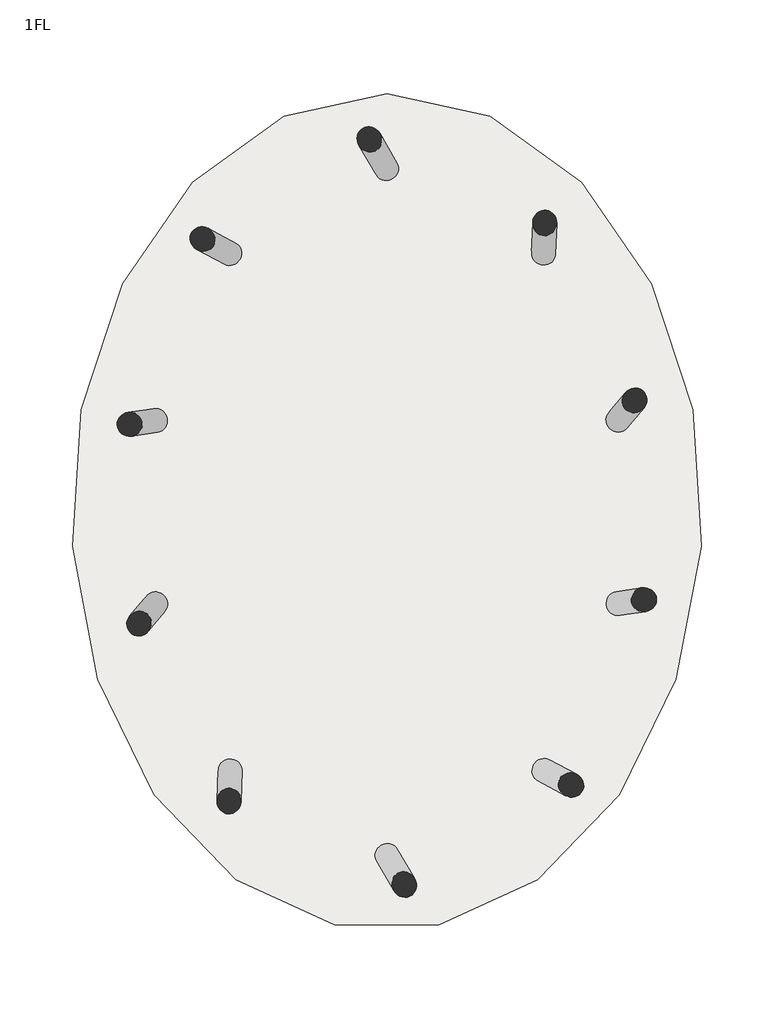
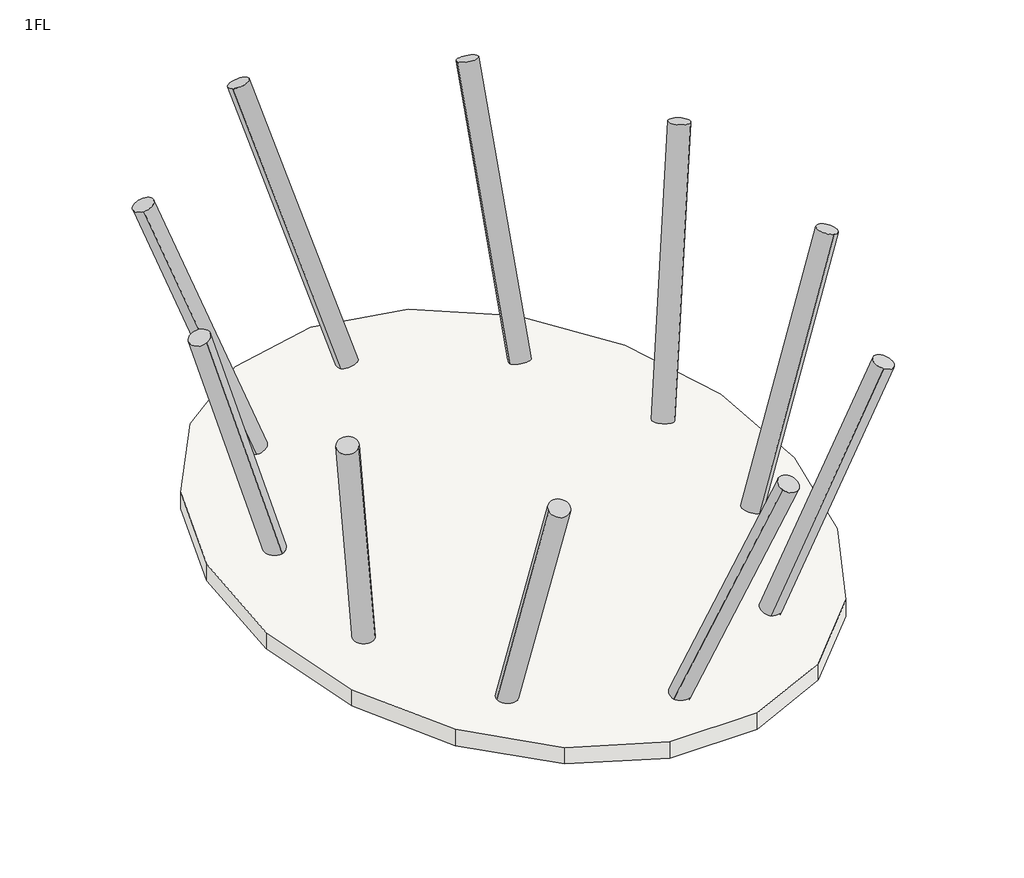
# One storey: 10 columns, 1 slab.
"""IFC4 building model written with IfcOpenShell, lengths in millimetres."""

import ifcopenshell
import ifcopenshell.guid

model = None  # the IFC model being written
_history = None  # IfcOwnerHistory: only IFC2X3 demands one
_inside = {}  # id of a spatial element -> (the spatial element, [elements in it])
_under = {}  # id of a project, library or spatial element -> (it, [spatial elements below it])
_declared = {}  # id of a project -> (the project, [libraries it declares])
_typed = {}  # id of a type object -> (the type object, [elements of that type])
_made_of = {}  # id of a material, layer set ... -> (it, [elements and type objects made of it])


def new_model(schema):
    """Start an empty IFC model of exactly this schema.

    Asked for "IFC4X3", IfcOpenShell would pick the latest addendum, in which some entities
    have other attributes; the version numbers below select the first issue.
    IFC2X3 requires an IfcOwnerHistory on every rooted entity: one is made here for all.
    """
    global model, _history
    if schema == "IFC4X3":
        model = ifcopenshell.file(schema_version=(4, 3, 0, 0))
    else:
        model = ifcopenshell.file(schema=schema)
    _inside.clear()
    _under.clear()
    _declared.clear()
    _typed.clear()
    _made_of.clear()
    _history = None
    if model.schema == "IFC2X3":
        org = make("IfcOrganization", Name="unknown")
        user = make(
            "IfcPersonAndOrganization",
            ThePerson=make("IfcPerson", FamilyName="unknown"),
            TheOrganization=org,
        )
        app = make(
            "IfcApplication",
            ApplicationDeveloper=org,
            Version="unknown",
            ApplicationFullName="unknown",
            ApplicationIdentifier="unknown",
        )
        _history = make(
            "IfcOwnerHistory",
            OwningUser=user,
            OwningApplication=app,
            ChangeAction="ADDED",
            CreationDate=0,
        )
    return model


def make(cls, **values):
    """One entity of the class cls with the attributes given. An attribute that is None is left unset."""
    return model.create_entity(
        cls, **{name: value for name, value in values.items() if value is not None}
    )


def rooted(cls, **values):
    """An entity with a GlobalId (a new one), such as an element, a storey or a relation."""
    return make(cls, GlobalId=ifcopenshell.guid.new(), OwnerHistory=_history, **values)


def si_unit(unit_type, name, prefix=None):
    """IfcSIUnit, for example si_unit("LENGTHUNIT", "METRE", prefix="MILLI")."""
    return make("IfcSIUnit", UnitType=unit_type, Prefix=prefix, Name=name)


def assignment(units):
    """IfcUnitAssignment: the units of a project."""
    return None if units is None else make("IfcUnitAssignment", Units=units)


def point(xyz):
    """IfcCartesianPoint."""
    return None if xyz is None else make("IfcCartesianPoint", Coordinates=xyz)


def direction(xyz):
    """IfcDirection."""
    return None if xyz is None else make("IfcDirection", DirectionRatios=xyz)


def frame(location, z_axis=None, x_axis=None):
    """IfcAxis2Placement3D, a coordinate frame: its origin and axes. An axis left out is left unset."""
    return make(
        "IfcAxis2Placement3D",
        Location=point(location),
        Axis=direction(z_axis),
        RefDirection=direction(x_axis),
    )


def frame_2d(location, x_axis=None):
    """IfcAxis2Placement2D, a coordinate frame in the plane: its origin and x axis."""
    return make(
        "IfcAxis2Placement2D", Location=point(location), RefDirection=direction(x_axis)
    )


def origin():
    """The frame at (0, 0, 0) with its axes left unset."""
    return frame((0.0, 0.0, 0.0))


def place(relative_to, where):
    """IfcLocalPlacement: puts the frame where relative to a parent placement (None: the world)."""
    return make(
        "IfcLocalPlacement", PlacementRelTo=relative_to, RelativePlacement=where
    )


def context(
    kind, dimensions, precision=None, world=None, true_north=None, identifier=None
):
    """IfcGeometricRepresentationContext, for example the 3D "Model" context."""
    return make(
        "IfcGeometricRepresentationContext",
        ContextIdentifier=identifier,
        ContextType=kind,
        CoordinateSpaceDimension=dimensions,
        Precision=precision,
        WorldCoordinateSystem=world,
        TrueNorth=true_north,
    )


def project(units=None, contexts=None):
    """IfcProject with its units and contexts."""
    return rooted(
        "IfcProject",
        Name="project",
        RepresentationContexts=contexts,
        UnitsInContext=assignment(units),
    )


def spatial(cls, under=None, at=None, **own):
    """A site, building, storey or space (cls), placed at a placement, below another one or the project."""
    s = rooted(cls, ObjectPlacement=at, **own)
    if under is not None:
        _under.setdefault(under.id(), (under, []))[1].append(s)
    return s


def polyline(points):
    """IfcPolyline through the points."""
    return make("IfcPolyline", Points=[point(p) for p in points])


def circle_curve(where, radius):
    """IfcCircle in the frame where."""
    return make("IfcCircle", Position=where, Radius=radius)


def trimmed(basis, trim1, trim2, sense, master):
    """IfcTrimmedCurve: the piece of a basis curve between two trims."""
    return make(
        "IfcTrimmedCurve",
        BasisCurve=basis,
        Trim1=trim1,
        Trim2=trim2,
        SenseAgreement=sense,
        MasterRepresentation=master,
    )


def segment(curve, same_sense, transition):
    """IfcCompositeCurveSegment."""
    return make(
        "IfcCompositeCurveSegment",
        Transition=transition,
        SameSense=same_sense,
        ParentCurve=curve,
    )


def composite_curve(segments, self_intersect=None):
    """IfcCompositeCurve: segments joined end to end."""
    return make("IfcCompositeCurve", Segments=segments, SelfIntersect=self_intersect)


def outline(outer, holes=None, kind="AREA"):
    """IfcArbitraryClosedProfileDef: a profile drawn as a closed curve; with holes, ...WithVoids."""
    if holes is None:
        return make("IfcArbitraryClosedProfileDef", ProfileType=kind, OuterCurve=outer)
    return make(
        "IfcArbitraryProfileDefWithVoids",
        ProfileType=kind,
        OuterCurve=outer,
        InnerCurves=holes,
    )


def extrude(swept, where, along, depth):
    """IfcExtrudedAreaSolid: the profile swept, set in the frame where, extruded along a direction by depth."""
    return make(
        "IfcExtrudedAreaSolid",
        SweptArea=swept,
        Position=where,
        ExtrudedDirection=direction(along),
        Depth=depth,
    )


def shape(context_of_items, identifier, shape_type, items):
    """IfcShapeRepresentation: the items that make up one representation, for example the "Body"."""
    return make(
        "IfcShapeRepresentation",
        ContextOfItems=context_of_items,
        RepresentationIdentifier=identifier,
        RepresentationType=shape_type,
        Items=items,
    )


def made_of(thing, what):
    """Note that an element or type object is made of a material, layer set ...; save() writes the relation."""
    if what is not None:
        _made_of.setdefault(what.id(), (what, []))[1].append(thing)
    return thing


def element(
    cls,
    number,
    at=None,
    inside=None,
    cuts=None,
    type_object=None,
    material=None,
    context=None,
    identifier="Body",
    shape_type=None,
    held_by="IfcProductDefinitionShape",
    body=None,
    shapes=None,
    **own,
):
    """One element of the class cls, such as IfcWall. Its Tag is "e" and its number.

    at: its placement. inside: the storey or other place that contains it. cuts: it is an
    opening in that element (IfcRelVoidsElement). A single representation is given by context,
    identifier, shape_type and body (its items); several are given by shapes. held_by: the class
    of the entity that holds the representations. save() writes the other relations.
    """
    e = rooted(cls, Tag="e%d" % number, ObjectPlacement=at, **own)
    if body is not None:
        shapes = [shape(context, identifier, shape_type, body)]
    if shapes is not None:
        e.Representation = make(held_by, Representations=shapes)
    if inside is not None:
        _inside.setdefault(inside.id(), (inside, []))[1].append(e)
    if cuts is not None:
        rooted(
            "IfcRelVoidsElement", RelatingBuildingElement=cuts, RelatedOpeningElement=e
        )
    if type_object is not None:
        _typed.setdefault(type_object.id(), (type_object, []))[1].append(e)
    return made_of(e, material)


def aggregate(whole, parts):
    """IfcRelAggregates: a whole, such as a stair, and the parts it consists of."""
    return rooted("IfcRelAggregates", RelatingObject=whole, RelatedObjects=parts)


def save(model, path):
    """Write the relations noted so far, then the file.

    IfcRelAggregates (storeys below a building ...), IfcRelContainedInSpatialStructure (elements
    in a storey), IfcRelDefinesByType, IfcRelAssociatesMaterial and IfcRelDeclares: one each for
    every whole, place, type object, material and project.
    """
    for whole, parts in _under.values():
        aggregate(whole, parts)
    for where, things in _inside.values():
        rooted(
            "IfcRelContainedInSpatialStructure",
            RelatedElements=things,
            RelatingStructure=where,
        )
    for kind, things in _typed.values():
        rooted("IfcRelDefinesByType", RelatedObjects=things, RelatingType=kind)
    for what, things in _made_of.values():
        rooted("IfcRelAssociatesMaterial", RelatedObjects=things, RelatingMaterial=what)
    for by, libraries in _declared.values():
        rooted("IfcRelDeclares", RelatingContext=by, RelatedDefinitions=libraries)
    model.write(path)


model = new_model("IFC4")

# Units and contexts
model_context = context("Model", 3, world=origin())
ifc_project = project(units=[si_unit("LENGTHUNIT", "METRE", prefix="MILLI")], contexts=[model_context])

# Site, building, storey
site = spatial("IfcSite", under=ifc_project)
building = spatial("IfcBuilding", under=site)
storey = spatial("IfcBuildingStorey", under=building, Name="1FL", Elevation=0.0)

# Columns
placement = place(None, origin())
element("IfcColumn", 1, ObjectType="コンクリート-円形-柱 : 750", at=placement, inside=storey, context=model_context, shape_type="SweptSolid", body=[
    extrude(outline(composite_curve([segment(trimmed(circle_curve(frame_2d((0.0, -175.0)), 175.0), [point((0.0, -350.0))], [point((0.0, 0.0))], False, "CARTESIAN"), True, "CONTINUOUS"), segment(trimmed(circle_curve(frame_2d((0.0, -175.0)), 175.0), [point((0.0, 0.0))], [point((0.0, -350.0))], False, "CARTESIAN"), True, "CONTINUOUS")], self_intersect=False)), frame((-150.9258136, 4911.4200994, 0.0), z_axis=(-0.19521767954583844, 0.33261932920084286, 0.9226345102123157), x_axis=(-0.46701070397496863, 0.7957106520636279, -0.3856754601543639)), (0.0, 0.0, 1.0), 4877.3376133),
])
element("IfcColumn", 2, ObjectType="コンクリート-円形-柱 : 750", at=placement, inside=storey, context=model_context, shape_type="SweptSolid", body=[
    extrude(outline(composite_curve([segment(trimmed(circle_curve(frame_2d((0.0, -175.0)), 175.0), [point((0.0, -350.0))], [point((0.0, 0.0))], False, "CARTESIAN"), True, "CONTINUOUS"), segment(trimmed(circle_curve(frame_2d((0.0, -175.0)), 175.0), [point((0.0, 0.0))], [point((0.0, -350.0))], False, "CARTESIAN"), True, "CONTINUOUS")], self_intersect=False)), frame((-2368.4341263, 3611.4937667, 0.0), z_axis=(-0.31275000049064827, 0.16672714276809913, 0.9350879622032815), x_axis=(-0.82515741745174, 0.43989172927194287, -0.3544157205070263)), (0.0, 0.0, 1.0), 4812.3814891),
])
element("IfcColumn", 3, ObjectType="コンクリート-円形-柱 : 750", at=placement, inside=storey, context=model_context, shape_type="SweptSolid", body=[
    extrude(outline(composite_curve([segment(trimmed(circle_curve(frame_2d((0.0, -175.0)), 175.0), [point((0.0, -350.0))], [point((0.0, 0.0))], False, "CARTESIAN"), True, "CONTINUOUS"), segment(trimmed(circle_curve(frame_2d((0.0, -175.0)), 175.0), [point((0.0, 0.0))], [point((0.0, -350.0))], False, "CARTESIAN"), True, "CONTINUOUS")], self_intersect=False)), frame((-3345.1996857, 1162.0255056, 0.0), z_axis=(-0.3023035165099614, -0.04397439962353301, 0.9521968473395936), x_axis=(-0.9422797649541056, -0.1370681605680071, -0.3054851287976858)), (0.0, 0.0, 1.0), 4725.9135677),
])
element("IfcColumn", 4, ObjectType="コンクリート-円形-柱 : 750", at=placement, inside=storey, context=model_context, shape_type="SweptSolid", body=[
    extrude(outline(composite_curve([segment(trimmed(circle_curve(frame_2d((0.0, -175.0)), 175.0), [point((0.0, -350.0))], [point((0.0, 0.0))], False, "CARTESIAN"), True, "CONTINUOUS"), segment(trimmed(circle_curve(frame_2d((0.0, -175.0)), 175.0), [point((0.0, 0.0))], [point((0.0, -350.0))], False, "CARTESIAN"), True, "CONTINUOUS")], self_intersect=False)), frame((-3236.0228376, -1447.3199745, 0.0), z_axis=(-0.19412294990655402, -0.23264885127893398, 0.9529904471284956), x_axis=(-0.6105515101907361, -0.7317223829581693, -0.3030003427090967)), (0.0, 0.0, 1.0), 4721.9780769),
])
element("IfcColumn", 5, ObjectType="コンクリート-円形-柱 : 750", at=placement, inside=storey, context=model_context, shape_type="SweptSolid", body=[
    extrude(outline(composite_curve([segment(trimmed(circle_curve(frame_2d((1e-07, -174.9999999)), 175.0), [point((0.0, -350.0))], [point((0.0, 0.0))], False, "CARTESIAN"), True, "CONTINUOUS"), segment(trimmed(circle_curve(frame_2d((1e-07, -174.9999999)), 175.0), [point((0.0, 0.0))], [point((0.0, -350.0))], False, "CARTESIAN"), True, "CONTINUOUS")], self_intersect=False)), frame((-2111.2371006, -3772.6097673, 0.0), z_axis=(-0.013415524296277117, -0.3507099157361099, 0.9363880492147616), x_axis=(-0.03579298830242224, -0.935703714164163, -0.3509664104836434)), (0.0, 0.0, 1.0), 4805.6999531),
])
element("IfcColumn", 6, ObjectType="コンクリート-円形-柱 : 750", at=placement, inside=storey, context=model_context, shape_type="SweptSolid", body=[
    extrude(outline(composite_curve([segment(trimmed(circle_curve(frame_2d((0.0, -175.0)), 175.0), [point((0.0, -349.9999999))], [point((0.0, 0.0))], False, "CARTESIAN"), True, "CONTINUOUS"), segment(trimmed(circle_curve(frame_2d((0.0, -175.0)), 175.0), [point((0.0, 0.0))], [point((0.0, -349.9999999))], False, "CARTESIAN"), True, "CONTINUOUS")], self_intersect=False)), frame((150.9258121, -4911.4201056, 0.0), z_axis=(0.19521768641578116, -0.332619328176475, 0.9226345091280188), x_axis=(0.46701071671984423, -0.7957106433262771, -0.3856754627482799)), (0.0, 0.0, 1.0), 4877.3376133),
])
element("IfcColumn", 7, ObjectType="コンクリート-円形-柱 : 750", at=placement, inside=storey, context=model_context, shape_type="SweptSolid", body=[
    extrude(outline(composite_curve([segment(trimmed(circle_curve(frame_2d((0.0, -175.0000001)), 175.0), [point((0.0, -350.0000001))], [point((0.0, 0.0))], False, "CARTESIAN"), True, "CONTINUOUS"), segment(trimmed(circle_curve(frame_2d((0.0, -175.0000001)), 175.0), [point((0.0, 0.0))], [point((0.0, -350.0000001))], False, "CARTESIAN"), True, "CONTINUOUS")], self_intersect=False)), frame((2368.4341596, -3611.4937481, 0.0), z_axis=(0.31274999648711344, -0.16672714070730643, 0.9350879639097471), x_axis=(0.8251574188770966, -0.439891730225705, -0.35441571600469896)), (0.0, 0.0, 1.0), 4812.3814891),
])
element("IfcColumn", 8, ObjectType="コンクリート-円形-柱 : 750", at=placement, inside=storey, context=model_context, shape_type="SweptSolid", body=[
    extrude(outline(composite_curve([segment(trimmed(circle_curve(frame_2d((-1e-07, -175.0000001)), 175.0), [point((0.0, -350.0))], [point((0.0, 0.0))], False, "CARTESIAN"), True, "CONTINUOUS"), segment(trimmed(circle_curve(frame_2d((-1e-07, -175.0000001)), 175.0), [point((0.0, 0.0))], [point((0.0, -350.0))], False, "CARTESIAN"), True, "CONTINUOUS")], self_intersect=False)), frame((3345.1996858, -1162.0254697, 0.0), z_axis=(0.30230351342511225, 0.04397439856797863, 0.9521968483677193), x_axis=(0.9422797662409613, 0.13706815886374568, -0.3054851255930188)), (0.0, 0.0, 1.0), 4725.9135677),
])
element("IfcColumn", 9, ObjectType="コンクリート-円形-柱 : 750", at=placement, inside=storey, context=model_context, shape_type="SweptSolid", body=[
    extrude(outline(composite_curve([segment(trimmed(circle_curve(frame_2d((0.0, -175.0)), 175.0), [point((0.0, -350.0))], [point((0.0, 0.0))], False, "CARTESIAN"), True, "CONTINUOUS"), segment(trimmed(circle_curve(frame_2d((0.0, -175.0)), 175.0), [point((0.0, 0.0))], [point((0.0, -350.0))], False, "CARTESIAN"), True, "CONTINUOUS")], self_intersect=False)), frame((3236.0228326, 1447.3200092, 0.0), z_axis=(0.19412294921583048, 0.23264884982996348, 0.9529904476229252), x_axis=(0.6105515114685474, 0.7317223825359012, -0.30300034115402713)), (0.0, 0.0, 1.0), 4721.9780769),
])
element("IfcColumn", 10, ObjectType="コンクリート-円形-柱 : 750", at=placement, inside=storey, context=model_context, shape_type="SweptSolid", body=[
    extrude(outline(composite_curve([segment(trimmed(circle_curve(frame_2d((-1e-07, -174.9999999)), 175.0), [point((-1e-07, -349.9999999))], [point((0.0, 0.0))], False, "CARTESIAN"), True, "CONTINUOUS"), segment(trimmed(circle_curve(frame_2d((-1e-07, -174.9999999)), 175.0), [point((0.0, 0.0))], [point((-1e-07, -349.9999999))], False, "CARTESIAN"), True, "CONTINUOUS")], self_intersect=False)), frame((2111.2370684, 3772.6097859, 0.0), z_axis=(0.013415528275215879, 0.3507099167842728, 0.9363880487651822), x_axis=(0.035792998778826544, 0.9357037133135062, -0.35096641168313336)), (0.0, 0.0, 1.0), 4805.6999531),
])

# Slab
element("IfcSlab", 11, ObjectType="一般 300 mm", at=placement, inside=storey, context=model_context, shape_type="SweptSolid", body=[
    extrude(outline(polyline([(-2836.452922, 4805.8475796), (-1502.9644736, 5768.0447322), (0.0, 6102.4452816), (1502.9644736, 5768.0447322), (2836.452922, 4805.8475796), (3857.7342177, 3326.6379287), (4461.3110743, 1491.9490879), (4585.2163062, -501.8023767), (4216.7090813, -2442.0718509), (3393.6531504, -4121.7797181), (2200.6194616, -5359.8802161), (762.4747723, -6018.1678182), (-762.4747709, -6018.1678065), (-2200.6194637, -5359.8802227), (-3393.653151, -4121.779719), (-4216.7090922, -2442.0718571), (-4585.2163041, -501.8023759), (-4461.311077, 1491.9490886), (-3857.7342176, 3326.6379288), (-2836.452922, 4805.8475796)])), frame((0.0, 0.0, -300.0), z_axis=(0.0, 0.0, 1.0), x_axis=(1.0, 0.0, 0.0)), (0.0, 0.0, 1.0), 300.0),
])

save(model, "model.ifc")

# Revit data of these elements
# Project information
#   プロジェクト発行日 = "発行日"
#   プロジェクト ステータス = "プロジェクト ステータス"
#   クライアント名 = "オーナ"
#   計画地住所 = "ここにアドレスを入力"
#   プロジェクト名 = "プロジェクト名"
#   プロジェクト番号 = "0001"
# Type "コンクリート-円形-柱 : 750"
#   Keynote = "03310.Q1"
#   R = 350 mm
#   Structural Material [instance default] = コンクリート - 現場打ち
# Type "一般 300 mm"
#   Function = 0
#   Layers, outside or top first: 300 mm no material (function 1)
# Elements 1, 2, 3, 4, 5, 6, 7, 8, 9, 10 (IfcColumn, "コンクリート-円形-柱 : 750")
#   Structural Material = コンクリート - 現場打ち
#   Phase Created = 新しい建設
#   Materials on its faces: "コンクリート - 現場打ち"
# Element 11 (IfcSlab, "一般 300 mm")
#   Height Offset From Level = 0 mm
#   Phase Created = 新しい建設
# Materials
#   "コンクリート - 現場打ち": class "コンクリート", colour RGB 192 192 192, transparency 0
